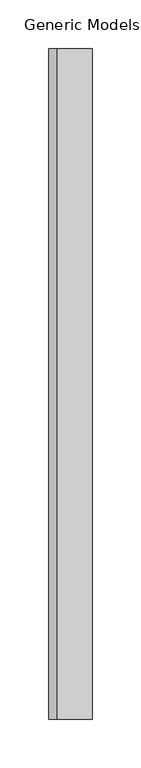
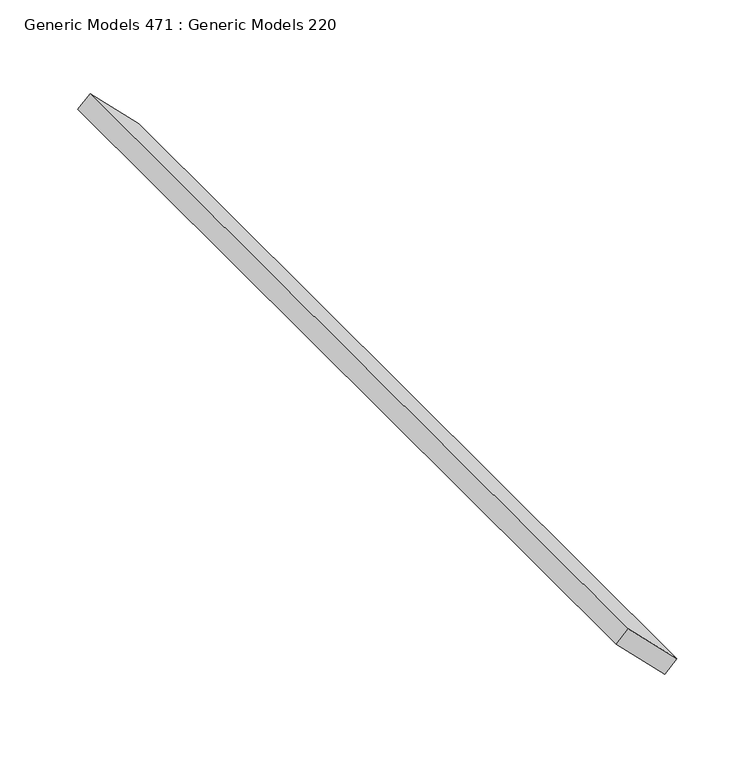
"""IFC4 building model written with IfcOpenShell, lengths in millimetres: proxy geometry, Generic Models 471 : Generic Models 220."""

import ifcopenshell
import ifcopenshell.guid

model = None  # the IFC model being written
_history = None  # IfcOwnerHistory: only IFC2X3 demands one
_inside = {}  # id of a spatial element -> (the spatial element, [elements in it])
_under = {}  # id of a project, library or spatial element -> (it, [spatial elements below it])
_declared = {}  # id of a project -> (the project, [libraries it declares])
_typed = {}  # id of a type object -> (the type object, [elements of that type])
_made_of = {}  # id of a material, layer set ... -> (it, [elements and type objects made of it])


def new_model(schema):
    """Start an empty IFC model of exactly this schema.

    Asked for "IFC4X3", IfcOpenShell would pick the latest addendum, in which some entities
    have other attributes; the version numbers below select the first issue.
    IFC2X3 requires an IfcOwnerHistory on every rooted entity: one is made here for all.
    """
    global model, _history
    if schema == "IFC4X3":
        model = ifcopenshell.file(schema_version=(4, 3, 0, 0))
    else:
        model = ifcopenshell.file(schema=schema)
    _inside.clear()
    _under.clear()
    _declared.clear()
    _typed.clear()
    _made_of.clear()
    _history = None
    if model.schema == "IFC2X3":
        org = make("IfcOrganization", Name="unknown")
        user = make(
            "IfcPersonAndOrganization",
            ThePerson=make("IfcPerson", FamilyName="unknown"),
            TheOrganization=org,
        )
        app = make(
            "IfcApplication",
            ApplicationDeveloper=org,
            Version="unknown",
            ApplicationFullName="unknown",
            ApplicationIdentifier="unknown",
        )
        _history = make(
            "IfcOwnerHistory",
            OwningUser=user,
            OwningApplication=app,
            ChangeAction="ADDED",
            CreationDate=0,
        )
    return model


def make(cls, **values):
    """One entity of the class cls with the attributes given. An attribute that is None is left unset."""
    return model.create_entity(
        cls, **{name: value for name, value in values.items() if value is not None}
    )


def rooted(cls, **values):
    """An entity with a GlobalId (a new one), such as an element, a storey or a relation."""
    return make(cls, GlobalId=ifcopenshell.guid.new(), OwnerHistory=_history, **values)


def si_unit(unit_type, name, prefix=None):
    """IfcSIUnit, for example si_unit("LENGTHUNIT", "METRE", prefix="MILLI")."""
    return make("IfcSIUnit", UnitType=unit_type, Prefix=prefix, Name=name)


def assignment(units):
    """IfcUnitAssignment: the units of a project."""
    return None if units is None else make("IfcUnitAssignment", Units=units)


def point(xyz):
    """IfcCartesianPoint."""
    return None if xyz is None else make("IfcCartesianPoint", Coordinates=xyz)


def direction(xyz):
    """IfcDirection."""
    return None if xyz is None else make("IfcDirection", DirectionRatios=xyz)


def frame(location, z_axis=None, x_axis=None):
    """IfcAxis2Placement3D, a coordinate frame: its origin and axes. An axis left out is left unset."""
    return make(
        "IfcAxis2Placement3D",
        Location=point(location),
        Axis=direction(z_axis),
        RefDirection=direction(x_axis),
    )


def origin():
    """The frame at (0, 0, 0) with its axes left unset."""
    return frame((0.0, 0.0, 0.0))


def place(relative_to, where):
    """IfcLocalPlacement: puts the frame where relative to a parent placement (None: the world)."""
    return make(
        "IfcLocalPlacement", PlacementRelTo=relative_to, RelativePlacement=where
    )


def context(
    kind, dimensions, precision=None, world=None, true_north=None, identifier=None
):
    """IfcGeometricRepresentationContext, for example the 3D "Model" context."""
    return make(
        "IfcGeometricRepresentationContext",
        ContextIdentifier=identifier,
        ContextType=kind,
        CoordinateSpaceDimension=dimensions,
        Precision=precision,
        WorldCoordinateSystem=world,
        TrueNorth=true_north,
    )


def project(units=None, contexts=None):
    """IfcProject with its units and contexts."""
    return rooted(
        "IfcProject",
        Name="project",
        RepresentationContexts=contexts,
        UnitsInContext=assignment(units),
    )


def spatial(cls, under=None, at=None, **own):
    """A site, building, storey or space (cls), placed at a placement, below another one or the project."""
    s = rooted(cls, ObjectPlacement=at, **own)
    if under is not None:
        _under.setdefault(under.id(), (under, []))[1].append(s)
    return s


def polyline(points):
    """IfcPolyline through the points."""
    return make("IfcPolyline", Points=[point(p) for p in points])


def outline(outer, holes=None, kind="AREA"):
    """IfcArbitraryClosedProfileDef: a profile drawn as a closed curve; with holes, ...WithVoids."""
    if holes is None:
        return make("IfcArbitraryClosedProfileDef", ProfileType=kind, OuterCurve=outer)
    return make(
        "IfcArbitraryProfileDefWithVoids",
        ProfileType=kind,
        OuterCurve=outer,
        InnerCurves=holes,
    )


def extrude(swept, where, along, depth):
    """IfcExtrudedAreaSolid: the profile swept, set in the frame where, extruded along a direction by depth."""
    return make(
        "IfcExtrudedAreaSolid",
        SweptArea=swept,
        Position=where,
        ExtrudedDirection=direction(along),
        Depth=depth,
    )


def shape(context_of_items, identifier, shape_type, items):
    """IfcShapeRepresentation: the items that make up one representation, for example the "Body"."""
    return make(
        "IfcShapeRepresentation",
        ContextOfItems=context_of_items,
        RepresentationIdentifier=identifier,
        RepresentationType=shape_type,
        Items=items,
    )


def source(mapping_origin, context_of_items, identifier, shape_type, items):
    """IfcRepresentationMap: a shape defined once, which mapped items show again and again."""
    return make(
        "IfcRepresentationMap",
        MappingOrigin=mapping_origin,
        MappedRepresentation=shape(context_of_items, identifier, shape_type, items),
    )


def transform(
    local_origin,
    x_axis=None,
    y_axis=None,
    z_axis=None,
    scale=None,
    scale2=None,
    scale3=None,
    uniform=True,
):
    """IfcCartesianTransformationOperator3D, or its non-uniform kind. x_axis, y_axis, z_axis: its Axis1, 2, 3."""
    if uniform:
        return make(
            "IfcCartesianTransformationOperator3D",
            Axis1=direction(x_axis),
            Axis2=direction(y_axis),
            LocalOrigin=point(local_origin),
            Scale=scale,
            Axis3=direction(z_axis),
        )
    return make(
        "IfcCartesianTransformationOperator3DnonUniform",
        Axis1=direction(x_axis),
        Axis2=direction(y_axis),
        LocalOrigin=point(local_origin),
        Scale=scale,
        Axis3=direction(z_axis),
        Scale2=scale2,
        Scale3=scale3,
    )


def mapped(mapping_source, mapping_target):
    """IfcMappedItem: shows the shape of a source again, moved by a transform."""
    return make(
        "IfcMappedItem", MappingSource=mapping_source, MappingTarget=mapping_target
    )


def made_of(thing, what):
    """Note that an element or type object is made of a material, layer set ...; save() writes the relation."""
    if what is not None:
        _made_of.setdefault(what.id(), (what, []))[1].append(thing)
    return thing


def element(
    cls,
    number,
    at=None,
    inside=None,
    cuts=None,
    type_object=None,
    material=None,
    context=None,
    identifier="Body",
    shape_type=None,
    held_by="IfcProductDefinitionShape",
    body=None,
    shapes=None,
    **own,
):
    """One element of the class cls, such as IfcWall. Its Tag is "e" and its number.

    at: its placement. inside: the storey or other place that contains it. cuts: it is an
    opening in that element (IfcRelVoidsElement). A single representation is given by context,
    identifier, shape_type and body (its items); several are given by shapes. held_by: the class
    of the entity that holds the representations. save() writes the other relations.
    """
    e = rooted(cls, Tag="e%d" % number, ObjectPlacement=at, **own)
    if body is not None:
        shapes = [shape(context, identifier, shape_type, body)]
    if shapes is not None:
        e.Representation = make(held_by, Representations=shapes)
    if inside is not None:
        _inside.setdefault(inside.id(), (inside, []))[1].append(e)
    if cuts is not None:
        rooted(
            "IfcRelVoidsElement", RelatingBuildingElement=cuts, RelatedOpeningElement=e
        )
    if type_object is not None:
        _typed.setdefault(type_object.id(), (type_object, []))[1].append(e)
    return made_of(e, material)


def aggregate(whole, parts):
    """IfcRelAggregates: a whole, such as a stair, and the parts it consists of."""
    return rooted("IfcRelAggregates", RelatingObject=whole, RelatedObjects=parts)


def save(model, path):
    """Write the relations noted so far, then the file.

    IfcRelAggregates (storeys below a building ...), IfcRelContainedInSpatialStructure (elements
    in a storey), IfcRelDefinesByType, IfcRelAssociatesMaterial and IfcRelDeclares: one each for
    every whole, place, type object, material and project.
    """
    for whole, parts in _under.values():
        aggregate(whole, parts)
    for where, things in _inside.values():
        rooted(
            "IfcRelContainedInSpatialStructure",
            RelatedElements=things,
            RelatingStructure=where,
        )
    for kind, things in _typed.values():
        rooted("IfcRelDefinesByType", RelatedObjects=things, RelatingType=kind)
    for what, things in _made_of.values():
        rooted("IfcRelAssociatesMaterial", RelatedObjects=things, RelatingMaterial=what)
    for by, libraries in _declared.values():
        rooted("IfcRelDeclares", RelatingContext=by, RelatedDefinitions=libraries)
    model.write(path)


def generic_models_471_generic_models_220_13c7f001(model_context):
    return source(origin(), model_context, "Body", "SweptSolid", [
        extrude(outline(polyline([(0.0, -50.8), (0.0, 0.0), (690.8142348, 0.0), (690.8142348, -50.8), (0.0, -50.8)])), frame((-6899.085451, -4564.8872686, 128132.6762561), z_axis=(0.7071067811865582, 0.0, 0.7071067811865369), x_axis=(0.0, 1.0, 0.0)), (0.0, 0.0, 1.0), 12.7),
    ])


if __name__ == "__main__":
    model = new_model("IFC4")
    model_context = context("Model", 3, world=origin())
    ifc_project = project(units=[si_unit("LENGTHUNIT", "METRE", prefix="MILLI")], contexts=[model_context])
    site = spatial("IfcSite", under=ifc_project)
    building = spatial("IfcBuilding", under=site)
    placement = place(None, origin())
    generic_models_471_generic_models_220_shape = generic_models_471_generic_models_220_13c7f001(model_context)
    element("IfcBuildingElementProxy", 1, Name="Generic Models 471 : Generic Models 220", ObjectType="Generic Models 471 : Generic Models 220", at=placement, inside=building, context=model_context, shape_type="MappedRepresentation", body=[
        mapped(generic_models_471_generic_models_220_shape, transform((0.0, 0.0, 0.0), x_axis=(1.0, 0.0, 0.0), y_axis=(0.0, 1.0, 0.0), z_axis=(0.0, 0.0, 1.0))),
    ])
    save(model, "model.ifc")

# Revit data of these elements
# Element 1 (IfcBuildingElementProxy, "Generic Models 471 : Generic Models 220")
#   Materials on its faces: "_WOOD TONE ALUMINUM EXTRUSION SLAT BY KNOTWOOD"
# Materials
#   "_WOOD TONE ALUMINUM EXTRUSION SLAT BY KNOTWOOD": class "Generic", colour RGB 177 130 114, transparency 0, Cost = 0
